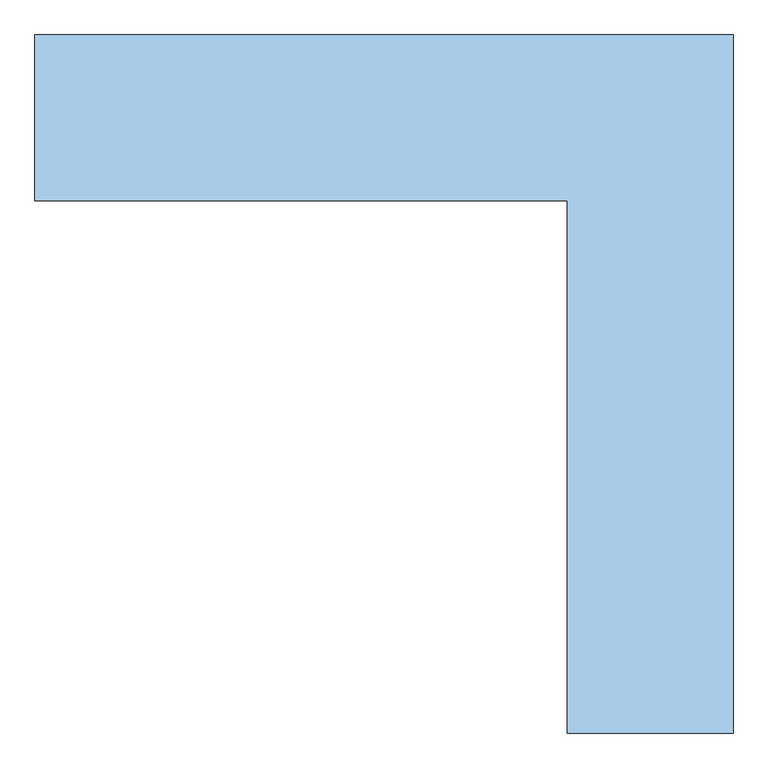
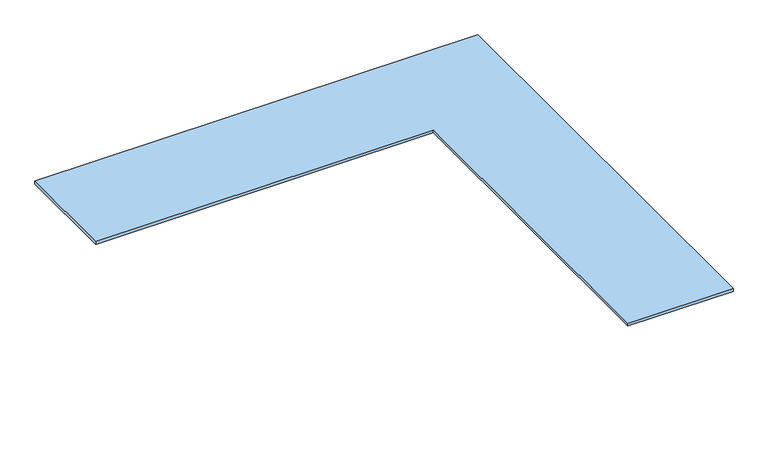
"""IFC4 building model written with IfcOpenShell, lengths in millimetres: window geometry, .CC_ND 300_PEDRA PEITORIL EM L : 3.06F x 3.06E x 0.73L."""

import ifcopenshell
import ifcopenshell.guid

model = None  # the IFC model being written
_history = None  # IfcOwnerHistory: only IFC2X3 demands one
_inside = {}  # id of a spatial element -> (the spatial element, [elements in it])
_under = {}  # id of a project, library or spatial element -> (it, [spatial elements below it])
_declared = {}  # id of a project -> (the project, [libraries it declares])
_typed = {}  # id of a type object -> (the type object, [elements of that type])
_made_of = {}  # id of a material, layer set ... -> (it, [elements and type objects made of it])


def new_model(schema):
    """Start an empty IFC model of exactly this schema.

    Asked for "IFC4X3", IfcOpenShell would pick the latest addendum, in which some entities
    have other attributes; the version numbers below select the first issue.
    IFC2X3 requires an IfcOwnerHistory on every rooted entity: one is made here for all.
    """
    global model, _history
    if schema == "IFC4X3":
        model = ifcopenshell.file(schema_version=(4, 3, 0, 0))
    else:
        model = ifcopenshell.file(schema=schema)
    _inside.clear()
    _under.clear()
    _declared.clear()
    _typed.clear()
    _made_of.clear()
    _history = None
    if model.schema == "IFC2X3":
        org = make("IfcOrganization", Name="unknown")
        user = make(
            "IfcPersonAndOrganization",
            ThePerson=make("IfcPerson", FamilyName="unknown"),
            TheOrganization=org,
        )
        app = make(
            "IfcApplication",
            ApplicationDeveloper=org,
            Version="unknown",
            ApplicationFullName="unknown",
            ApplicationIdentifier="unknown",
        )
        _history = make(
            "IfcOwnerHistory",
            OwningUser=user,
            OwningApplication=app,
            ChangeAction="ADDED",
            CreationDate=0,
        )
    return model


def make(cls, **values):
    """One entity of the class cls with the attributes given. An attribute that is None is left unset."""
    return model.create_entity(
        cls, **{name: value for name, value in values.items() if value is not None}
    )


def rooted(cls, **values):
    """An entity with a GlobalId (a new one), such as an element, a storey or a relation."""
    return make(cls, GlobalId=ifcopenshell.guid.new(), OwnerHistory=_history, **values)


def si_unit(unit_type, name, prefix=None):
    """IfcSIUnit, for example si_unit("LENGTHUNIT", "METRE", prefix="MILLI")."""
    return make("IfcSIUnit", UnitType=unit_type, Prefix=prefix, Name=name)


def assignment(units):
    """IfcUnitAssignment: the units of a project."""
    return None if units is None else make("IfcUnitAssignment", Units=units)


def point(xyz):
    """IfcCartesianPoint."""
    return None if xyz is None else make("IfcCartesianPoint", Coordinates=xyz)


def direction(xyz):
    """IfcDirection."""
    return None if xyz is None else make("IfcDirection", DirectionRatios=xyz)


def frame(location, z_axis=None, x_axis=None):
    """IfcAxis2Placement3D, a coordinate frame: its origin and axes. An axis left out is left unset."""
    return make(
        "IfcAxis2Placement3D",
        Location=point(location),
        Axis=direction(z_axis),
        RefDirection=direction(x_axis),
    )


def origin():
    """The frame at (0, 0, 0) with its axes left unset."""
    return frame((0.0, 0.0, 0.0))


def place(relative_to, where):
    """IfcLocalPlacement: puts the frame where relative to a parent placement (None: the world)."""
    return make(
        "IfcLocalPlacement", PlacementRelTo=relative_to, RelativePlacement=where
    )


def context(
    kind, dimensions, precision=None, world=None, true_north=None, identifier=None
):
    """IfcGeometricRepresentationContext, for example the 3D "Model" context."""
    return make(
        "IfcGeometricRepresentationContext",
        ContextIdentifier=identifier,
        ContextType=kind,
        CoordinateSpaceDimension=dimensions,
        Precision=precision,
        WorldCoordinateSystem=world,
        TrueNorth=true_north,
    )


def project(units=None, contexts=None):
    """IfcProject with its units and contexts."""
    return rooted(
        "IfcProject",
        Name="project",
        RepresentationContexts=contexts,
        UnitsInContext=assignment(units),
    )


def spatial(cls, under=None, at=None, **own):
    """A site, building, storey or space (cls), placed at a placement, below another one or the project."""
    s = rooted(cls, ObjectPlacement=at, **own)
    if under is not None:
        _under.setdefault(under.id(), (under, []))[1].append(s)
    return s


def polyline(points):
    """IfcPolyline through the points."""
    return make("IfcPolyline", Points=[point(p) for p in points])


def outline(outer, holes=None, kind="AREA"):
    """IfcArbitraryClosedProfileDef: a profile drawn as a closed curve; with holes, ...WithVoids."""
    if holes is None:
        return make("IfcArbitraryClosedProfileDef", ProfileType=kind, OuterCurve=outer)
    return make(
        "IfcArbitraryProfileDefWithVoids",
        ProfileType=kind,
        OuterCurve=outer,
        InnerCurves=holes,
    )


def extrude(swept, where, along, depth):
    """IfcExtrudedAreaSolid: the profile swept, set in the frame where, extruded along a direction by depth."""
    return make(
        "IfcExtrudedAreaSolid",
        SweptArea=swept,
        Position=where,
        ExtrudedDirection=direction(along),
        Depth=depth,
    )


def shape(context_of_items, identifier, shape_type, items):
    """IfcShapeRepresentation: the items that make up one representation, for example the "Body"."""
    return make(
        "IfcShapeRepresentation",
        ContextOfItems=context_of_items,
        RepresentationIdentifier=identifier,
        RepresentationType=shape_type,
        Items=items,
    )


def source(mapping_origin, context_of_items, identifier, shape_type, items):
    """IfcRepresentationMap: a shape defined once, which mapped items show again and again."""
    return make(
        "IfcRepresentationMap",
        MappingOrigin=mapping_origin,
        MappedRepresentation=shape(context_of_items, identifier, shape_type, items),
    )


def transform(
    local_origin,
    x_axis=None,
    y_axis=None,
    z_axis=None,
    scale=None,
    scale2=None,
    scale3=None,
    uniform=True,
):
    """IfcCartesianTransformationOperator3D, or its non-uniform kind. x_axis, y_axis, z_axis: its Axis1, 2, 3."""
    if uniform:
        return make(
            "IfcCartesianTransformationOperator3D",
            Axis1=direction(x_axis),
            Axis2=direction(y_axis),
            LocalOrigin=point(local_origin),
            Scale=scale,
            Axis3=direction(z_axis),
        )
    return make(
        "IfcCartesianTransformationOperator3DnonUniform",
        Axis1=direction(x_axis),
        Axis2=direction(y_axis),
        LocalOrigin=point(local_origin),
        Scale=scale,
        Axis3=direction(z_axis),
        Scale2=scale2,
        Scale3=scale3,
    )


def mapped(mapping_source, mapping_target):
    """IfcMappedItem: shows the shape of a source again, moved by a transform."""
    return make(
        "IfcMappedItem", MappingSource=mapping_source, MappingTarget=mapping_target
    )


def made_of(thing, what):
    """Note that an element or type object is made of a material, layer set ...; save() writes the relation."""
    if what is not None:
        _made_of.setdefault(what.id(), (what, []))[1].append(thing)
    return thing


def element(
    cls,
    number,
    at=None,
    inside=None,
    cuts=None,
    type_object=None,
    material=None,
    context=None,
    identifier="Body",
    shape_type=None,
    held_by="IfcProductDefinitionShape",
    body=None,
    shapes=None,
    **own,
):
    """One element of the class cls, such as IfcWall. Its Tag is "e" and its number.

    at: its placement. inside: the storey or other place that contains it. cuts: it is an
    opening in that element (IfcRelVoidsElement). A single representation is given by context,
    identifier, shape_type and body (its items); several are given by shapes. held_by: the class
    of the entity that holds the representations. save() writes the other relations.
    """
    e = rooted(cls, Tag="e%d" % number, ObjectPlacement=at, **own)
    if body is not None:
        shapes = [shape(context, identifier, shape_type, body)]
    if shapes is not None:
        e.Representation = make(held_by, Representations=shapes)
    if inside is not None:
        _inside.setdefault(inside.id(), (inside, []))[1].append(e)
    if cuts is not None:
        rooted(
            "IfcRelVoidsElement", RelatingBuildingElement=cuts, RelatedOpeningElement=e
        )
    if type_object is not None:
        _typed.setdefault(type_object.id(), (type_object, []))[1].append(e)
    return made_of(e, material)


def aggregate(whole, parts):
    """IfcRelAggregates: a whole, such as a stair, and the parts it consists of."""
    return rooted("IfcRelAggregates", RelatingObject=whole, RelatedObjects=parts)


def save(model, path):
    """Write the relations noted so far, then the file.

    IfcRelAggregates (storeys below a building ...), IfcRelContainedInSpatialStructure (elements
    in a storey), IfcRelDefinesByType, IfcRelAssociatesMaterial and IfcRelDeclares: one each for
    every whole, place, type object, material and project.
    """
    for whole, parts in _under.values():
        aggregate(whole, parts)
    for where, things in _inside.values():
        rooted(
            "IfcRelContainedInSpatialStructure",
            RelatedElements=things,
            RelatingStructure=where,
        )
    for kind, things in _typed.values():
        rooted("IfcRelDefinesByType", RelatedObjects=things, RelatingType=kind)
    for what, things in _made_of.values():
        rooted("IfcRelAssociatesMaterial", RelatedObjects=things, RelatingMaterial=what)
    for by, libraries in _declared.values():
        rooted("IfcRelDeclares", RelatingContext=by, RelatedDefinitions=libraries)
    model.write(path)


def window_829f86a1(model_context):
    return source(origin(), model_context, "Body", "SweptSolid", [
        extrude(outline(polyline([(-1265.0, -98.8), (-1265.0, 628.8), (1795.0, 628.8), (1795.0, -2431.2), (1067.4, -2431.2), (1067.4, -98.8), (-1265.0, -98.8)])), frame((0.0, 0.0, 900.0), z_axis=(0.0, 0.0, 1.0), x_axis=(1.0, 0.0, 0.0)), (0.0, 0.0, 1.0), 20.0),
    ])


if __name__ == "__main__":
    model = new_model("IFC4")
    model_context = context("Model", 3, world=origin())
    ifc_project = project(units=[si_unit("LENGTHUNIT", "METRE", prefix="MILLI")], contexts=[model_context])
    site = spatial("IfcSite", under=ifc_project)
    building = spatial("IfcBuilding", under=site)
    placement = place(None, origin())
    window_shape = window_829f86a1(model_context)
    element("IfcWindow", 1, ObjectType=".CC_ND 300_PEDRA PEITORIL EM L : 3.06F x 3.06E x 0.73L", at=placement, inside=building, context=model_context, shape_type="MappedRepresentation", body=[
        mapped(window_shape, transform((0.0, 0.0, 0.0), x_axis=(1.0, 0.0, 0.0), y_axis=(0.0, 1.0, 0.0), z_axis=(0.0, 0.0, 1.0))),
    ])
    save(model, "model.ifc")

# Revit data of these elements
# Type ".CC_ND 300_PEDRA PEITORIL EM L : 3.06F x 3.06E x 0.73L"
#   Type Mark = "63"
#   Largura da pedra da frente [instance default] = 0.26 m
#   Largura da pedra da esquerda [instance default] = 0.26 m
#   Extensão esquerda interna [instance default] = 0.03 m
#   Extensão esquerda externa [instance default] = 0.03 m
#   Comprimento Esquerda = 2.3324 m
#   Extensão frente interna [instance default] = 0.03 m
#   Extensão frente externa [instance default] = 0.03 m
#   Espessura peitoril = 0.02 m
#   Espessura da parede [instance default] = 0.20 m
#   Comprimento da pedra [instance default] = 4.8624 m
#   Comprimento Frente = 2.53 m
#   Altura-padrão do peitoril [instance default] = 0.90 m
#   Pedra do peitoril = .GRANITO_BRANCO_ITAUNAS
#   Rough Width = 0
#   Rough Height = 0
#   Height = 0
#   Wall Closure = (empty or 0)
#   Width = 0
# Element 1 (IfcWindow, ".CC_ND 300_PEDRA PEITORIL EM L : 3.06F x 3.06E x 0.73L")
#   Largura da pedra da frente = 0.7276 m
#   Largura da pedra da esquerda = 0.7276 m
#   Extensão esquerda interna = 0.00 m
#   Extensão esquerda externa = 0.53 m
#   Extensão frente interna = 0.00 m
#   Extensão frente externa = 0.53 m
#   Espessura da parede = 0.1976 m
#   Materials on its faces: ".GRANITO_BRANCO_ITAUNAS"
# Materials
#   ".GRANITO_BRANCO_ITAUNAS": class ".CC_PEDRA REVEST.", colour RGB 202 195 174, transparency 0, Description = "Revestimento em granito", Cost = 0
